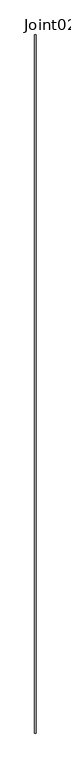
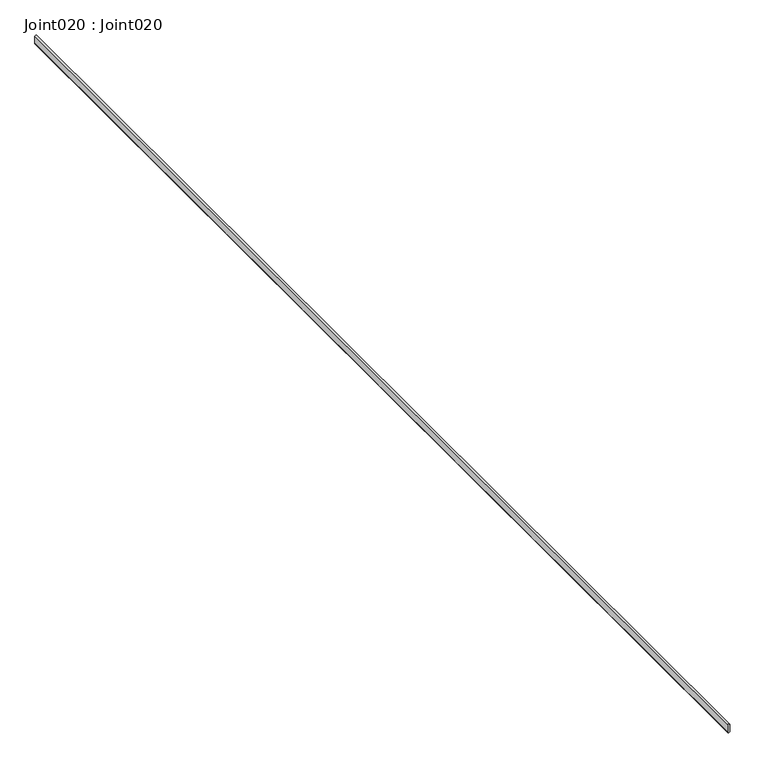
"""IFC4 building model written with IfcOpenShell, lengths in millimetres: proxy geometry, Joint020 : Joint020."""

from ifc_helpers import new_model, si_unit, point, frame, frame_2d, origin, place, context, project, spatial, polyline, circle_curve, trimmed, segment, composite_curve, outline, extrude, source, transform, mapped, element, save


def joint020_joint020_a2196c3a(model_context):
    return source(origin(), model_context, "Body", "SweptSolid", [
        extrude(outline(composite_curve([segment(polyline([(42123.2804083, -2456.7369768), (42111.2057013, -2456.7369768)]), True, "CONTINUOUS"), segment(trimmed(circle_curve(frame_2d((42111.2057013, -2454.9713518)), 1.765625), [point((42111.2057013, -2456.7369768))], [point((42111.2057013, -2453.2057268))], False, "CARTESIAN"), True, "CONTINUOUS"), segment(polyline([(42111.2057013, -2453.2057268), (42123.2804083, -2453.2057268)]), True, "CONTINUOUS"), segment(trimmed(circle_curve(frame_2d((42123.2804083, -2454.9713518)), 1.765625), [point((42123.2804083, -2453.2057268))], [point((42123.2804083, -2456.7369768))], False, "CARTESIAN"), True, "CONTINUOUS")], self_intersect=False)), frame((0.0, -1052.8906574, 0.0), z_axis=(0.0, 1.0, 0.0), x_axis=(0.0, 0.0, 1.0)), (0.0, 0.0, 1.0), 2000.0),
    ])


if __name__ == "__main__":
    model = new_model("IFC4")
    model_context = context("Model", 3, world=origin())
    ifc_project = project(units=[si_unit("LENGTHUNIT", "METRE", prefix="MILLI")], contexts=[model_context])
    site = spatial("IfcSite", under=ifc_project)
    building = spatial("IfcBuilding", under=site)
    placement = place(None, origin())
    joint020_joint020_shape = joint020_joint020_a2196c3a(model_context)
    element("IfcBuildingElementProxy", 1, Name="Joint020 : Joint020", ObjectType="Joint020 : Joint020", at=placement, inside=building, context=model_context, shape_type="MappedRepresentation", body=[
        mapped(joint020_joint020_shape, transform((0.0, 0.0, 0.0), x_axis=(1.0, 0.0, 0.0), y_axis=(0.0, 1.0, 0.0), z_axis=(0.0, 0.0, 1.0))),
    ])
    save(model, "model.ifc")

# Revit data of these elements
# Type "Joint020 : Joint020"
#   NameOverride = "Joint020"
# Element 1 (IfcBuildingElementProxy, "Joint020 : Joint020")
#   Materials on its faces: "SILICON JOINT"
# Materials
#   "SILICON JOINT": class "Unassigned", colour RGB 150 184 127, transparency 0
